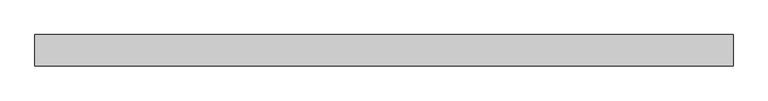
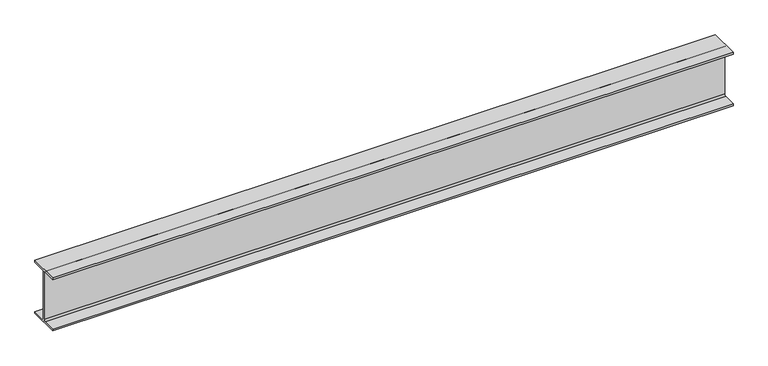
"""IFC4 building model written with IfcOpenShell, lengths in millimetres: beam geometry, Old_Steel Beam_H-KSD3502 : H_SB_ASB_H-200×200x8x12."""

from ifc_helpers import new_model, si_unit, point, frame, frame_2d, origin, place, context, project, spatial, polyline, circle_curve, trimmed, segment, composite_curve, outline, extrude, source, transform, mapped, element, save


def beam_fe90bdae(model_context):
    return source(origin(), model_context, "Body", "SweptSolid", [
        extrude(outline(composite_curve([segment(polyline([(82.5, -141.5), (82.5, -151.7), (-82.5, -151.7), (-82.5, -141.5), (-11.9, -141.5)]), True, "CONTINUOUS"), segment(trimmed(circle_curve(frame_2d((-11.9, -132.6)), 8.9), [point((-11.9, -141.5))], [point((-3.0, -132.6))], True, "CARTESIAN"), True, "CONTINUOUS"), segment(polyline([(-3.0, -132.6), (-3.0, 132.6)]), True, "CONTINUOUS"), segment(trimmed(circle_curve(frame_2d((-11.9, 132.6)), 8.9), [point((-3.0, 132.6))], [point((-11.9, 141.5))], True, "CARTESIAN"), True, "CONTINUOUS"), segment(polyline([(-11.9, 141.5), (-82.5, 141.5), (-82.5, 151.7), (82.5, 151.7), (82.5, 141.5), (11.9, 141.5)]), True, "CONTINUOUS"), segment(trimmed(circle_curve(frame_2d((11.9, 132.6)), 8.9), [point((11.9, 141.5))], [point((3.0, 132.6))], True, "CARTESIAN"), True, "CONTINUOUS"), segment(polyline([(3.0, 132.6), (3.0, -132.6)]), True, "CONTINUOUS"), segment(trimmed(circle_curve(frame_2d((11.9, -132.6)), 8.9), [point((3.0, -132.6))], [point((11.9, -141.5))], True, "CARTESIAN"), True, "CONTINUOUS"), segment(polyline([(11.9, -141.5), (82.5, -141.5)]), True, "CONTINUOUS")], self_intersect=False)), frame((-1848.779151, 0.0, 0.0), z_axis=(1.0, 0.0, 0.0), x_axis=(0.0, 1.0, 0.0)), (0.0, 0.0, 1.0), 3672.4688696),
    ])


if __name__ == "__main__":
    model = new_model("IFC4")
    model_context = context("Model", 3, world=origin())
    ifc_project = project(units=[si_unit("LENGTHUNIT", "METRE", prefix="MILLI")], contexts=[model_context])
    site = spatial("IfcSite", under=ifc_project)
    building = spatial("IfcBuilding", under=site)
    placement = place(None, origin())
    beam_shape = beam_fe90bdae(model_context)
    element("IfcBeam", 1, ObjectType="Old_Steel Beam_H-KSD3502 : H_SB_ASB_H-200×200x8x12", at=placement, inside=building, context=model_context, shape_type="MappedRepresentation", body=[
        mapped(beam_shape, transform((0.0, 0.0, 0.0), x_axis=(1.0, 0.0, 0.0), y_axis=(0.0, 1.0, 0.0), z_axis=(0.0, 0.0, 1.0))),
    ])
    save(model, "model.ifc")

# Revit data of these elements
# Type "Old_Steel Beam_H-KSD3502 : H_SB_ASB_H-200×200x8x12"
#   Width = 20.0 cm
#   Web Thickness = 0.8 cm
#   Web Fillet = 1.3 cm
#   Warping Constant = 141376.0 cm⁶
#   Torsional Moment of Inertia = 26.2485 cm⁴
#   Torsional Modulus = 1.0 cm³
#   Section Area = 63.53 cm²
#   Plastic Modulus weak axis = 244.0 cm³
#   Plastic Modulus strong axis = 525.0 cm³
#   Perimeter = 1.16 m²/m
#   Nominal Weight = 49.90 kgf/m
#   Moment of Inertia weak axis = 1600.00 cm⁴
#   Moment of Inertia strong axis = 4720.00 cm⁴
#   Height = 20.0 cm
#   Flange Thickness = 1.2 cm
#   Elastic Modulus weak axis = 160.0 cm³
#   Elastic Modulus strong axis = 472.0 cm³
#   Centroid Vertical = 10.0 cm
#   Centroid Horizontal = 10.0 cm
#   Length [instance default] = 1.5240 m
#   Structural Material [instance default] = Steel, 45-345
#   Assembly Code = ""
# Element 1 (IfcBeam, "Old_Steel Beam_H-KSD3502 : H_SB_ASB_H-200×200x8x12")
#   Structural Material = none
# Materials
#   "Steel, 45-345": class "Metal", colour RGB 189 187 185, transparency 0, Description = "Steel 345 MPa", Cost = 0
